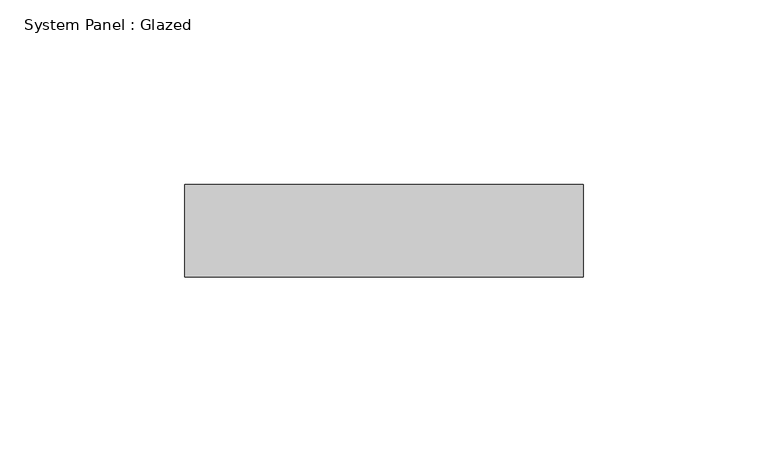
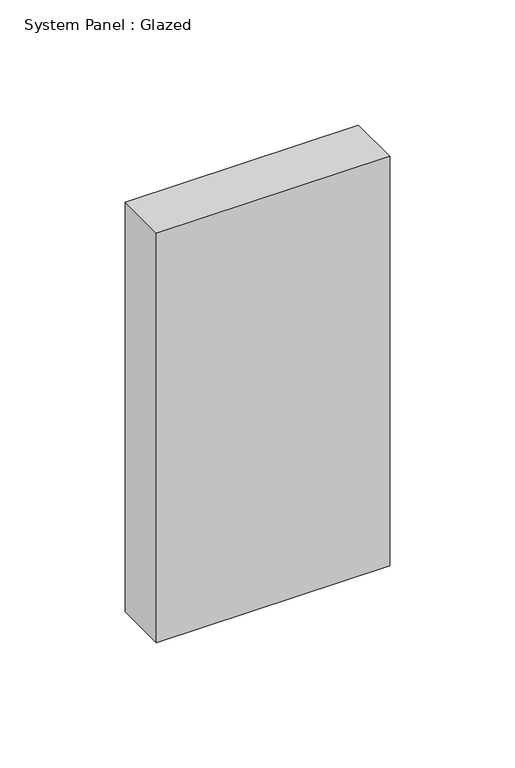
"""IFC4 building model written with IfcOpenShell, lengths in millimetres: plate geometry, System Panel : Glazed."""

from ifc_helpers import new_model, si_unit, origin, origin_with_axes, place, context, project, spatial, polyline, outline, extrude, source, transform, mapped, element, save


def system_panel_glazed_1c271f2e(model_context):
    return source(origin(), model_context, "Body", "SweptSolid", [
        extrude(outline(polyline([(53.879849, 24.5), (-53.879849, 24.5), (-53.879849, 49.5), (53.879849, 49.5), (53.879849, 24.5)])), origin_with_axes(), (0.0, 0.0, 1.0), 200.0),
    ])


if __name__ == "__main__":
    model = new_model("IFC4")
    model_context = context("Model", 3, world=origin())
    ifc_project = project(units=[si_unit("LENGTHUNIT", "METRE", prefix="MILLI")], contexts=[model_context])
    site = spatial("IfcSite", under=ifc_project)
    building = spatial("IfcBuilding", under=site)
    placement = place(None, origin())
    system_panel_glazed_shape = system_panel_glazed_1c271f2e(model_context)
    element("IfcPlate", 1, ObjectType="System Panel : Glazed", at=placement, inside=building, context=model_context, shape_type="MappedRepresentation", body=[
        mapped(system_panel_glazed_shape, transform((0.0, 0.0, 0.0), x_axis=(1.0, 0.0, 0.0), y_axis=(0.0, 1.0, 0.0), z_axis=(0.0, 0.0, 1.0))),
    ])
    save(model, "model.ifc")

# Revit data of these elements
# Element 1 (IfcPlate, "System Panel : Glazed")
#   Materials on its faces: "Glass"
# Materials
#   "Glass": class "Glass", colour RGB 218 227 224, transparency 0.85, Description = "Soda Lime Glass", Cost = 0
